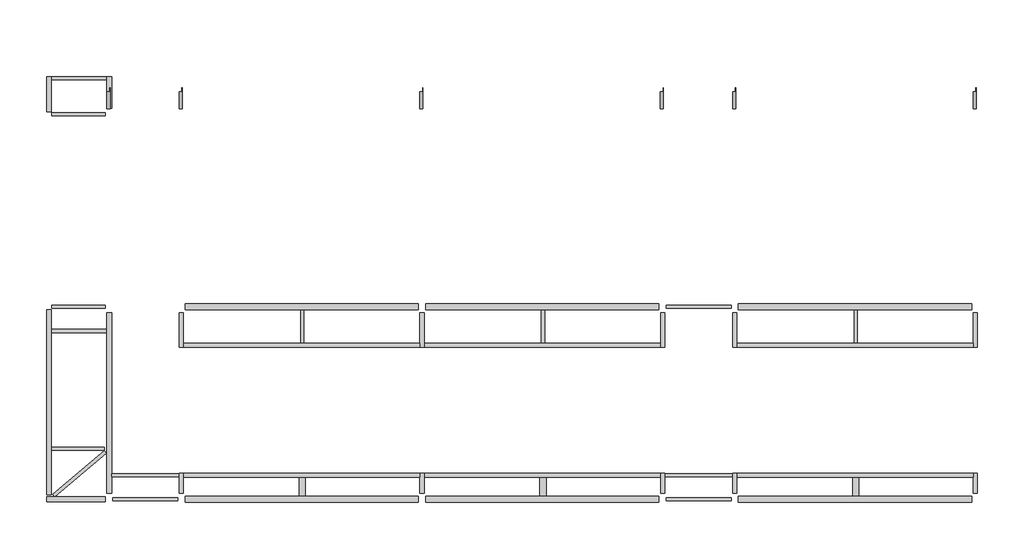
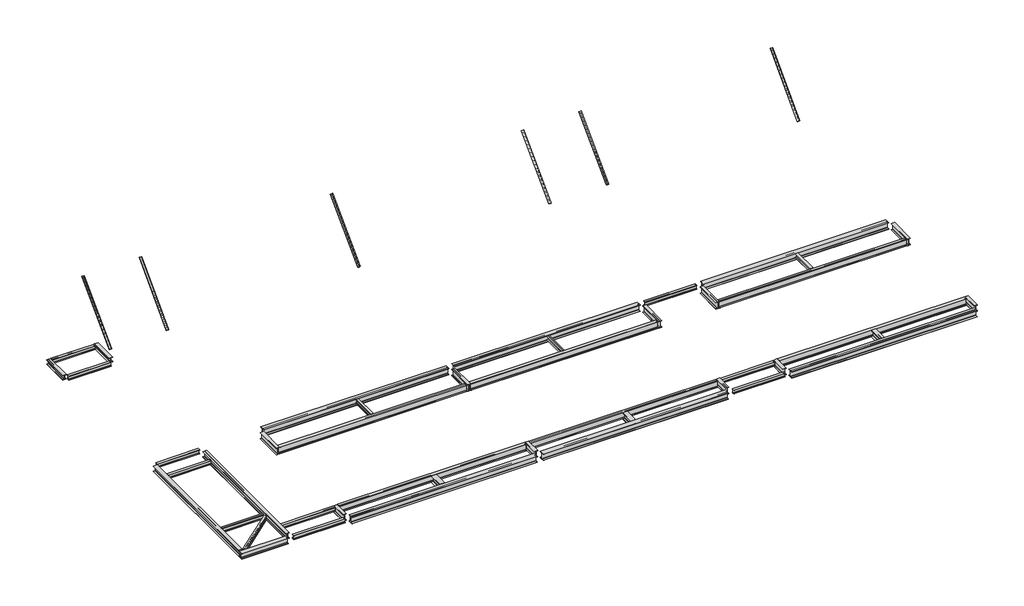
# One storey: 44 beams, 6 members.
"""IFC4 building model written with IfcOpenShell, lengths in millimetres."""

import ifcopenshell
import ifcopenshell.guid

model = None  # the IFC model being written
_history = None  # IfcOwnerHistory: only IFC2X3 demands one
_inside = {}  # id of a spatial element -> (the spatial element, [elements in it])
_under = {}  # id of a project, library or spatial element -> (it, [spatial elements below it])
_declared = {}  # id of a project -> (the project, [libraries it declares])
_typed = {}  # id of a type object -> (the type object, [elements of that type])
_made_of = {}  # id of a material, layer set ... -> (it, [elements and type objects made of it])


def new_model(schema):
    """Start an empty IFC model of exactly this schema.

    Asked for "IFC4X3", IfcOpenShell would pick the latest addendum, in which some entities
    have other attributes; the version numbers below select the first issue.
    IFC2X3 requires an IfcOwnerHistory on every rooted entity: one is made here for all.
    """
    global model, _history
    if schema == "IFC4X3":
        model = ifcopenshell.file(schema_version=(4, 3, 0, 0))
    else:
        model = ifcopenshell.file(schema=schema)
    _inside.clear()
    _under.clear()
    _declared.clear()
    _typed.clear()
    _made_of.clear()
    _history = None
    if model.schema == "IFC2X3":
        org = make("IfcOrganization", Name="unknown")
        user = make(
            "IfcPersonAndOrganization",
            ThePerson=make("IfcPerson", FamilyName="unknown"),
            TheOrganization=org,
        )
        app = make(
            "IfcApplication",
            ApplicationDeveloper=org,
            Version="unknown",
            ApplicationFullName="unknown",
            ApplicationIdentifier="unknown",
        )
        _history = make(
            "IfcOwnerHistory",
            OwningUser=user,
            OwningApplication=app,
            ChangeAction="ADDED",
            CreationDate=0,
        )
    return model


def make(cls, **values):
    """One entity of the class cls with the attributes given. An attribute that is None is left unset."""
    return model.create_entity(
        cls, **{name: value for name, value in values.items() if value is not None}
    )


def rooted(cls, **values):
    """An entity with a GlobalId (a new one), such as an element, a storey or a relation."""
    return make(cls, GlobalId=ifcopenshell.guid.new(), OwnerHistory=_history, **values)


def si_unit(unit_type, name, prefix=None):
    """IfcSIUnit, for example si_unit("LENGTHUNIT", "METRE", prefix="MILLI")."""
    return make("IfcSIUnit", UnitType=unit_type, Prefix=prefix, Name=name)


def assignment(units):
    """IfcUnitAssignment: the units of a project."""
    return None if units is None else make("IfcUnitAssignment", Units=units)


def point(xyz):
    """IfcCartesianPoint."""
    return None if xyz is None else make("IfcCartesianPoint", Coordinates=xyz)


def direction(xyz):
    """IfcDirection."""
    return None if xyz is None else make("IfcDirection", DirectionRatios=xyz)


def frame(location, z_axis=None, x_axis=None):
    """IfcAxis2Placement3D, a coordinate frame: its origin and axes. An axis left out is left unset."""
    return make(
        "IfcAxis2Placement3D",
        Location=point(location),
        Axis=direction(z_axis),
        RefDirection=direction(x_axis),
    )


def frame_2d(location, x_axis=None):
    """IfcAxis2Placement2D, a coordinate frame in the plane: its origin and x axis."""
    return make(
        "IfcAxis2Placement2D", Location=point(location), RefDirection=direction(x_axis)
    )


def origin():
    """The frame at (0, 0, 0) with its axes left unset."""
    return frame((0.0, 0.0, 0.0))


def place(relative_to, where):
    """IfcLocalPlacement: puts the frame where relative to a parent placement (None: the world)."""
    return make(
        "IfcLocalPlacement", PlacementRelTo=relative_to, RelativePlacement=where
    )


def context(
    kind, dimensions, precision=None, world=None, true_north=None, identifier=None
):
    """IfcGeometricRepresentationContext, for example the 3D "Model" context."""
    return make(
        "IfcGeometricRepresentationContext",
        ContextIdentifier=identifier,
        ContextType=kind,
        CoordinateSpaceDimension=dimensions,
        Precision=precision,
        WorldCoordinateSystem=world,
        TrueNorth=true_north,
    )


def project(units=None, contexts=None):
    """IfcProject with its units and contexts."""
    return rooted(
        "IfcProject",
        Name="project",
        RepresentationContexts=contexts,
        UnitsInContext=assignment(units),
    )


def spatial(cls, under=None, at=None, **own):
    """A site, building, storey or space (cls), placed at a placement, below another one or the project."""
    s = rooted(cls, ObjectPlacement=at, **own)
    if under is not None:
        _under.setdefault(under.id(), (under, []))[1].append(s)
    return s


def polyline(points):
    """IfcPolyline through the points."""
    return make("IfcPolyline", Points=[point(p) for p in points])


def circle_curve(where, radius):
    """IfcCircle in the frame where."""
    return make("IfcCircle", Position=where, Radius=radius)


def trimmed(basis, trim1, trim2, sense, master):
    """IfcTrimmedCurve: the piece of a basis curve between two trims."""
    return make(
        "IfcTrimmedCurve",
        BasisCurve=basis,
        Trim1=trim1,
        Trim2=trim2,
        SenseAgreement=sense,
        MasterRepresentation=master,
    )


def segment(curve, same_sense, transition):
    """IfcCompositeCurveSegment."""
    return make(
        "IfcCompositeCurveSegment",
        Transition=transition,
        SameSense=same_sense,
        ParentCurve=curve,
    )


def composite_curve(segments, self_intersect=None):
    """IfcCompositeCurve: segments joined end to end."""
    return make("IfcCompositeCurve", Segments=segments, SelfIntersect=self_intersect)


def outline(outer, holes=None, kind="AREA"):
    """IfcArbitraryClosedProfileDef: a profile drawn as a closed curve; with holes, ...WithVoids."""
    if holes is None:
        return make("IfcArbitraryClosedProfileDef", ProfileType=kind, OuterCurve=outer)
    return make(
        "IfcArbitraryProfileDefWithVoids",
        ProfileType=kind,
        OuterCurve=outer,
        InnerCurves=holes,
    )


def extrude(swept, where, along, depth):
    """IfcExtrudedAreaSolid: the profile swept, set in the frame where, extruded along a direction by depth."""
    return make(
        "IfcExtrudedAreaSolid",
        SweptArea=swept,
        Position=where,
        ExtrudedDirection=direction(along),
        Depth=depth,
    )


def shape(context_of_items, identifier, shape_type, items):
    """IfcShapeRepresentation: the items that make up one representation, for example the "Body"."""
    return make(
        "IfcShapeRepresentation",
        ContextOfItems=context_of_items,
        RepresentationIdentifier=identifier,
        RepresentationType=shape_type,
        Items=items,
    )


def source(mapping_origin, context_of_items, identifier, shape_type, items):
    """IfcRepresentationMap: a shape defined once, which mapped items show again and again."""
    return make(
        "IfcRepresentationMap",
        MappingOrigin=mapping_origin,
        MappedRepresentation=shape(context_of_items, identifier, shape_type, items),
    )


def transform(
    local_origin,
    x_axis=None,
    y_axis=None,
    z_axis=None,
    scale=None,
    scale2=None,
    scale3=None,
    uniform=True,
):
    """IfcCartesianTransformationOperator3D, or its non-uniform kind. x_axis, y_axis, z_axis: its Axis1, 2, 3."""
    if uniform:
        return make(
            "IfcCartesianTransformationOperator3D",
            Axis1=direction(x_axis),
            Axis2=direction(y_axis),
            LocalOrigin=point(local_origin),
            Scale=scale,
            Axis3=direction(z_axis),
        )
    return make(
        "IfcCartesianTransformationOperator3DnonUniform",
        Axis1=direction(x_axis),
        Axis2=direction(y_axis),
        LocalOrigin=point(local_origin),
        Scale=scale,
        Axis3=direction(z_axis),
        Scale2=scale2,
        Scale3=scale3,
    )


def mapped(mapping_source, mapping_target):
    """IfcMappedItem: shows the shape of a source again, moved by a transform."""
    return make(
        "IfcMappedItem", MappingSource=mapping_source, MappingTarget=mapping_target
    )


def made_of(thing, what):
    """Note that an element or type object is made of a material, layer set ...; save() writes the relation."""
    if what is not None:
        _made_of.setdefault(what.id(), (what, []))[1].append(thing)
    return thing


def element(
    cls,
    number,
    at=None,
    inside=None,
    cuts=None,
    type_object=None,
    material=None,
    context=None,
    identifier="Body",
    shape_type=None,
    held_by="IfcProductDefinitionShape",
    body=None,
    shapes=None,
    **own,
):
    """One element of the class cls, such as IfcWall. Its Tag is "e" and its number.

    at: its placement. inside: the storey or other place that contains it. cuts: it is an
    opening in that element (IfcRelVoidsElement). A single representation is given by context,
    identifier, shape_type and body (its items); several are given by shapes. held_by: the class
    of the entity that holds the representations. save() writes the other relations.
    """
    e = rooted(cls, Tag="e%d" % number, ObjectPlacement=at, **own)
    if body is not None:
        shapes = [shape(context, identifier, shape_type, body)]
    if shapes is not None:
        e.Representation = make(held_by, Representations=shapes)
    if inside is not None:
        _inside.setdefault(inside.id(), (inside, []))[1].append(e)
    if cuts is not None:
        rooted(
            "IfcRelVoidsElement", RelatingBuildingElement=cuts, RelatedOpeningElement=e
        )
    if type_object is not None:
        _typed.setdefault(type_object.id(), (type_object, []))[1].append(e)
    return made_of(e, material)


def aggregate(whole, parts):
    """IfcRelAggregates: a whole, such as a stair, and the parts it consists of."""
    return rooted("IfcRelAggregates", RelatingObject=whole, RelatedObjects=parts)


def save(model, path):
    """Write the relations noted so far, then the file.

    IfcRelAggregates (storeys below a building ...), IfcRelContainedInSpatialStructure (elements
    in a storey), IfcRelDefinesByType, IfcRelAssociatesMaterial and IfcRelDeclares: one each for
    every whole, place, type object, material and project.
    """
    for whole, parts in _under.values():
        aggregate(whole, parts)
    for where, things in _inside.values():
        rooted(
            "IfcRelContainedInSpatialStructure",
            RelatedElements=things,
            RelatingStructure=where,
        )
    for kind, things in _typed.values():
        rooted("IfcRelDefinesByType", RelatedObjects=things, RelatingType=kind)
    for what, things in _made_of.values():
        rooted("IfcRelAssociatesMaterial", RelatedObjects=things, RelatingMaterial=what)
    for by, libraries in _declared.values():
        rooted("IfcRelDeclares", RelatingContext=by, RelatedDefinitions=libraries)
    model.write(path)


def steel_framing_w_astm_a6m_f33feb28(model_context):
    return source(origin(), model_context, "Body", "SweptSolid", [
        extrude(outline(composite_curve([segment(polyline([(67.0, -94.8), (67.0, -105.0), (-67.0, -105.0), (-67.0, -94.8), (-10.775, -94.8)]), True, "CONTINUOUS"), segment(trimmed(circle_curve(frame_2d((-10.775, -87.2)), 7.6), [point((-10.775, -94.8))], [point((-3.175, -87.2))], True, "CARTESIAN"), True, "CONTINUOUS"), segment(polyline([(-3.175, -87.2), (-3.175, 87.2)]), True, "CONTINUOUS"), segment(trimmed(circle_curve(frame_2d((-10.775, 87.2)), 7.6), [point((-3.175, 87.2))], [point((-10.775, 94.8))], True, "CARTESIAN"), True, "CONTINUOUS"), segment(polyline([(-10.775, 94.8), (-67.0, 94.8), (-67.0, 105.0), (67.0, 105.0), (67.0, 94.8), (10.775, 94.8)]), True, "CONTINUOUS"), segment(trimmed(circle_curve(frame_2d((10.775, 87.2)), 7.6), [point((10.775, 94.8))], [point((3.175, 87.2))], True, "CARTESIAN"), True, "CONTINUOUS"), segment(polyline([(3.175, 87.2), (3.175, -87.2)]), True, "CONTINUOUS"), segment(trimmed(circle_curve(frame_2d((10.775, -87.2)), 7.6), [point((3.175, -87.2))], [point((10.775, -94.8))], True, "CARTESIAN"), True, "CONTINUOUS"), segment(polyline([(10.775, -94.8), (67.0, -94.8)]), True, "CONTINUOUS")], self_intersect=False)), frame((-1346.3, 0.0, 0.0), z_axis=(1.0, 0.0, 0.0), x_axis=(0.0, 1.0, 0.0)), (0.0, 0.0, 1.0), 2692.6),
    ])


def steel_framing_w_astm_a6m_9ad7bea0(model_context):
    return source(origin(), model_context, "Body", "SweptSolid", [
        extrude(outline(composite_curve([segment(polyline([(67.0, -94.8), (67.0, -105.0), (-67.0, -105.0), (-67.0, -94.8), (-10.775, -94.8)]), True, "CONTINUOUS"), segment(trimmed(circle_curve(frame_2d((-10.775, -87.2)), 7.6), [point((-10.775, -94.8))], [point((-3.175, -87.2))], True, "CARTESIAN"), True, "CONTINUOUS"), segment(polyline([(-3.175, -87.2), (-3.175, 87.2)]), True, "CONTINUOUS"), segment(trimmed(circle_curve(frame_2d((-10.775, 87.2)), 7.6), [point((-3.175, 87.2))], [point((-10.775, 94.8))], True, "CARTESIAN"), True, "CONTINUOUS"), segment(polyline([(-10.775, 94.8), (-67.0, 94.8), (-67.0, 105.0), (67.0, 105.0), (67.0, 94.8), (10.775, 94.8)]), True, "CONTINUOUS"), segment(trimmed(circle_curve(frame_2d((10.775, 87.2)), 7.6), [point((10.775, 94.8))], [point((3.175, 87.2))], True, "CARTESIAN"), True, "CONTINUOUS"), segment(polyline([(3.175, 87.2), (3.175, -87.2)]), True, "CONTINUOUS"), segment(trimmed(circle_curve(frame_2d((10.775, -87.2)), 7.6), [point((3.175, -87.2))], [point((10.775, -94.8))], True, "CARTESIAN"), True, "CONTINUOUS"), segment(polyline([(10.775, -94.8), (67.0, -94.8)]), True, "CONTINUOUS")], self_intersect=False)), frame((-1135.3, 0.0, 0.0), z_axis=(1.0, 0.0, 0.0), x_axis=(0.0, 1.0, 0.0)), (0.0, 0.0, 1.0), 2231.6),
    ])


def steel_framing_w_astm_a6m_5f95f2a9(model_context):
    return source(origin(), model_context, "Body", "SweptSolid", [
        extrude(outline(composite_curve([segment(polyline([(67.0, -94.8), (67.0, -105.0), (-67.0, -105.0), (-67.0, -94.8), (-10.775, -94.8)]), True, "CONTINUOUS"), segment(trimmed(circle_curve(frame_2d((-10.775, -87.2)), 7.6), [point((-10.775, -94.8))], [point((-3.175, -87.2))], True, "CARTESIAN"), True, "CONTINUOUS"), segment(polyline([(-3.175, -87.2), (-3.175, 87.2)]), True, "CONTINUOUS"), segment(trimmed(circle_curve(frame_2d((-10.775, 87.2)), 7.6), [point((-3.175, 87.2))], [point((-10.775, 94.8))], True, "CARTESIAN"), True, "CONTINUOUS"), segment(polyline([(-10.775, 94.8), (-67.0, 94.8), (-67.0, 105.0), (67.0, 105.0), (67.0, 94.8), (10.775, 94.8)]), True, "CONTINUOUS"), segment(trimmed(circle_curve(frame_2d((10.775, 87.2)), 7.6), [point((10.775, 94.8))], [point((3.175, 87.2))], True, "CARTESIAN"), True, "CONTINUOUS"), segment(polyline([(3.175, 87.2), (3.175, -87.2)]), True, "CONTINUOUS"), segment(trimmed(circle_curve(frame_2d((10.775, -87.2)), 7.6), [point((3.175, -87.2))], [point((10.775, -94.8))], True, "CARTESIAN"), True, "CONTINUOUS"), segment(polyline([(10.775, -94.8), (67.0, -94.8)]), True, "CONTINUOUS")], self_intersect=False)), frame((-1401.8, 0.0, 0.0), z_axis=(1.0, 0.0, 0.0), x_axis=(0.0, 1.0, 0.0)), (0.0, 0.0, 1.0), 2803.6),
    ])


def steel_framing_w_astm_a6m_17837fc5(model_context):
    return source(origin(), model_context, "Body", "SweptSolid", [
        extrude(outline(composite_curve([segment(polyline([(127.0, -160.1), (127.0, -176.5), (-127.0, -176.5), (-127.0, -160.1), (-19.865, -160.1)]), True, "CONTINUOUS"), segment(trimmed(circle_curve(frame_2d((-19.865, -145.0)), 15.1), [point((-19.865, -160.1))], [point((-4.765, -145.0))], True, "CARTESIAN"), True, "CONTINUOUS"), segment(polyline([(-4.765, -145.0), (-4.765, 145.0)]), True, "CONTINUOUS"), segment(trimmed(circle_curve(frame_2d((-19.865, 145.0)), 15.1), [point((-4.765, 145.0))], [point((-19.865, 160.1))], True, "CARTESIAN"), True, "CONTINUOUS"), segment(polyline([(-19.865, 160.1), (-127.0, 160.1), (-127.0, 176.5), (127.0, 176.5), (127.0, 160.1), (19.865, 160.1)]), True, "CONTINUOUS"), segment(trimmed(circle_curve(frame_2d((19.865, 145.0)), 15.1), [point((19.865, 160.1))], [point((4.765, 145.0))], True, "CARTESIAN"), True, "CONTINUOUS"), segment(polyline([(4.765, 145.0), (4.765, -145.0)]), True, "CONTINUOUS"), segment(trimmed(circle_curve(frame_2d((19.865, -145.0)), 15.1), [point((4.765, -145.0))], [point((19.865, -160.1))], True, "CARTESIAN"), True, "CONTINUOUS"), segment(polyline([(19.865, -160.1), (127.0, -160.1)]), True, "CONTINUOUS")], self_intersect=False)), frame((-4846.3, 0.0, 0.0), z_axis=(1.0, 0.0, 0.0), x_axis=(0.0, 1.0, 0.0)), (0.0, 0.0, 1.0), 9692.6),
    ])


def steel_framing_w_astm_a6m_8cea9429(model_context):
    return source(origin(), model_context, "Body", "SweptSolid", [
        extrude(outline(composite_curve([segment(polyline([(101.5, -137.9), (101.5, -151.0), (-101.5, -151.0), (-101.5, -137.9), (-16.545, -137.9)]), True, "CONTINUOUS"), segment(trimmed(circle_curve(frame_2d((-16.545, -125.1)), 12.8), [point((-16.545, -137.9))], [point((-3.745, -125.1))], True, "CARTESIAN"), True, "CONTINUOUS"), segment(polyline([(-3.745, -125.1), (-3.745, 125.1)]), True, "CONTINUOUS"), segment(trimmed(circle_curve(frame_2d((-16.545, 125.1)), 12.8), [point((-3.745, 125.1))], [point((-16.545, 137.9))], True, "CARTESIAN"), True, "CONTINUOUS"), segment(polyline([(-16.545, 137.9), (-101.5, 137.9), (-101.5, 151.0), (101.5, 151.0), (101.5, 137.9), (16.545, 137.9)]), True, "CONTINUOUS"), segment(trimmed(circle_curve(frame_2d((16.545, 125.1)), 12.8), [point((16.545, 137.9))], [point((3.745, 125.1))], True, "CARTESIAN"), True, "CONTINUOUS"), segment(polyline([(3.745, 125.1), (3.745, -125.1)]), True, "CONTINUOUS"), segment(trimmed(circle_curve(frame_2d((16.545, -125.1)), 12.8), [point((3.745, -125.1))], [point((16.545, -137.9))], True, "CARTESIAN"), True, "CONTINUOUS"), segment(polyline([(16.545, -137.9), (101.5, -137.9)]), True, "CONTINUOUS")], self_intersect=False)), frame((-3753.8, 0.0, 0.0), z_axis=(1.0, 0.0, 0.0), x_axis=(0.0, 1.0, 0.0)), (0.0, 0.0, 1.0), 7507.6),
    ])


def steel_framing_w_astm_a6m_ee6b765e(model_context):
    return source(origin(), model_context, "Body", "SweptSolid", [
        extrude(outline(composite_curve([segment(polyline([(101.0, -112.5), (101.0, -123.5), (-101.0, -123.5), (-101.0, -112.5), (-16.385, -112.5)]), True, "CONTINUOUS"), segment(trimmed(circle_curve(frame_2d((-16.385, -99.8)), 12.7), [point((-16.385, -112.5))], [point((-3.685, -99.8))], True, "CARTESIAN"), True, "CONTINUOUS"), segment(polyline([(-3.685, -99.8), (-3.685, 99.8)]), True, "CONTINUOUS"), segment(trimmed(circle_curve(frame_2d((-16.385, 99.8)), 12.7), [point((-3.685, 99.8))], [point((-16.385, 112.5))], True, "CARTESIAN"), True, "CONTINUOUS"), segment(polyline([(-16.385, 112.5), (-101.0, 112.5), (-101.0, 123.5), (101.0, 123.5), (101.0, 112.5), (16.385, 112.5)]), True, "CONTINUOUS"), segment(trimmed(circle_curve(frame_2d((16.385, 99.8)), 12.7), [point((16.385, 112.5))], [point((3.685, 99.8))], True, "CARTESIAN"), True, "CONTINUOUS"), segment(polyline([(3.685, 99.8), (3.685, -99.8)]), True, "CONTINUOUS"), segment(trimmed(circle_curve(frame_2d((16.385, -99.8)), 12.7), [point((3.685, -99.8))], [point((16.385, -112.5))], True, "CARTESIAN"), True, "CONTINUOUS"), segment(polyline([(16.385, -112.5), (101.0, -112.5)]), True, "CONTINUOUS")], self_intersect=False)), frame((-634.3, 0.0, 0.0), z_axis=(1.0, 0.0, 0.0), x_axis=(0.0, 1.0, 0.0)), (0.0, 0.0, 1.0), 1451.3),
    ])


def steel_framing_w_astm_a6m_8355ed91(model_context):
    return source(origin(), model_context, "Body", "SweptSolid", [
        extrude(outline(composite_curve([segment(polyline([(67.0, -94.8), (67.0, -105.0), (-67.0, -105.0), (-67.0, -94.8), (-10.775, -94.8)]), True, "CONTINUOUS"), segment(trimmed(circle_curve(frame_2d((-10.775, -87.2)), 7.6), [point((-10.775, -94.8))], [point((-3.175, -87.2))], True, "CARTESIAN"), True, "CONTINUOUS"), segment(polyline([(-3.175, -87.2), (-3.175, 87.2)]), True, "CONTINUOUS"), segment(trimmed(circle_curve(frame_2d((-10.775, 87.2)), 7.6), [point((-3.175, 87.2))], [point((-10.775, 94.8))], True, "CARTESIAN"), True, "CONTINUOUS"), segment(polyline([(-10.775, 94.8), (-67.0, 94.8), (-67.0, 105.0), (67.0, 105.0), (67.0, 94.8), (10.775, 94.8)]), True, "CONTINUOUS"), segment(trimmed(circle_curve(frame_2d((10.775, 87.2)), 7.6), [point((10.775, 94.8))], [point((3.175, 87.2))], True, "CARTESIAN"), True, "CONTINUOUS"), segment(polyline([(3.175, 87.2), (3.175, -87.2)]), True, "CONTINUOUS"), segment(trimmed(circle_curve(frame_2d((10.775, -87.2)), 7.6), [point((3.175, -87.2))], [point((10.775, -94.8))], True, "CARTESIAN"), True, "CONTINUOUS"), segment(polyline([(10.775, -94.8), (67.0, -94.8)]), True, "CONTINUOUS")], self_intersect=False)), frame((-1136.3, 0.0, 0.0), z_axis=(1.0, 0.0, 0.0), x_axis=(0.0, 1.0, 0.0)), (0.0, 0.0, 1.0), 2272.6),
    ])


def steel_framing_w_astm_a6m_7f0d9279(model_context):
    return source(origin(), model_context, "Body", "SweptSolid", [
        extrude(outline(composite_curve([segment(polyline([(101.0, -112.5), (101.0, -123.5), (-101.0, -123.5), (-101.0, -112.5), (-16.385, -112.5)]), True, "CONTINUOUS"), segment(trimmed(circle_curve(frame_2d((-16.385, -99.8)), 12.7), [point((-16.385, -112.5))], [point((-3.685, -99.8))], True, "CARTESIAN"), True, "CONTINUOUS"), segment(polyline([(-3.685, -99.8), (-3.685, 99.8)]), True, "CONTINUOUS"), segment(trimmed(circle_curve(frame_2d((-16.385, 99.8)), 12.7), [point((-3.685, 99.8))], [point((-16.385, 112.5))], True, "CARTESIAN"), True, "CONTINUOUS"), segment(polyline([(-16.385, 112.5), (-101.0, 112.5), (-101.0, 123.5), (101.0, 123.5), (101.0, 112.5), (16.385, 112.5)]), True, "CONTINUOUS"), segment(trimmed(circle_curve(frame_2d((16.385, 99.8)), 12.7), [point((16.385, 112.5))], [point((3.685, 99.8))], True, "CARTESIAN"), True, "CONTINUOUS"), segment(polyline([(3.685, 99.8), (3.685, -99.8)]), True, "CONTINUOUS"), segment(trimmed(circle_curve(frame_2d((16.385, -99.8)), 12.7), [point((3.685, -99.8))], [point((16.385, -112.5))], True, "CARTESIAN"), True, "CONTINUOUS"), segment(polyline([(16.385, -112.5), (101.0, -112.5)]), True, "CONTINUOUS")], self_intersect=False)), frame((-503.8, 0.0, 0.0), z_axis=(1.0, 0.0, 0.0), x_axis=(0.0, 1.0, 0.0)), (0.0, 0.0, 1.0), 1320.8),
    ])


def steel_framing_w_astm_a6m_9f313648(model_context):
    return source(origin(), model_context, "Body", "SweptSolid", [
        extrude(outline(composite_curve([segment(polyline([(67.0, -94.8), (67.0, -105.0), (-67.0, -105.0), (-67.0, -94.8), (-10.775, -94.8)]), True, "CONTINUOUS"), segment(trimmed(circle_curve(frame_2d((-10.775, -87.2)), 7.6), [point((-10.775, -94.8))], [point((-3.175, -87.2))], True, "CARTESIAN"), True, "CONTINUOUS"), segment(polyline([(-3.175, -87.2), (-3.175, 87.2)]), True, "CONTINUOUS"), segment(trimmed(circle_curve(frame_2d((-10.775, 87.2)), 7.6), [point((-3.175, 87.2))], [point((-10.775, 94.8))], True, "CARTESIAN"), True, "CONTINUOUS"), segment(polyline([(-10.775, 94.8), (-67.0, 94.8), (-67.0, 105.0), (67.0, 105.0), (67.0, 94.8), (10.775, 94.8)]), True, "CONTINUOUS"), segment(trimmed(circle_curve(frame_2d((10.775, 87.2)), 7.6), [point((10.775, 94.8))], [point((3.175, 87.2))], True, "CARTESIAN"), True, "CONTINUOUS"), segment(polyline([(3.175, 87.2), (3.175, -87.2)]), True, "CONTINUOUS"), segment(trimmed(circle_curve(frame_2d((10.775, -87.2)), 7.6), [point((3.175, -87.2))], [point((10.775, -94.8))], True, "CARTESIAN"), True, "CONTINUOUS"), segment(polyline([(10.775, -94.8), (67.0, -94.8)]), True, "CONTINUOUS")], self_intersect=False)), frame((-1135.8, 0.0, 0.0), z_axis=(1.0, 0.0, 0.0), x_axis=(0.0, 1.0, 0.0)), (0.0, 0.0, 1.0), 2271.6),
    ])


def steel_framing_w_astm_a6m_8815720a(model_context):
    return source(origin(), model_context, "Body", "SweptSolid", [
        extrude(outline(composite_curve([segment(polyline([(101.5, -137.9), (101.5, -151.0), (-101.5, -151.0), (-101.5, -137.9), (-16.545, -137.9)]), True, "CONTINUOUS"), segment(trimmed(circle_curve(frame_2d((-16.545, -125.1)), 12.8), [point((-16.545, -137.9))], [point((-3.745, -125.1))], True, "CARTESIAN"), True, "CONTINUOUS"), segment(polyline([(-3.745, -125.1), (-3.745, 125.1)]), True, "CONTINUOUS"), segment(trimmed(circle_curve(frame_2d((-16.545, 125.1)), 12.8), [point((-3.745, 125.1))], [point((-16.545, 137.9))], True, "CARTESIAN"), True, "CONTINUOUS"), segment(polyline([(-16.545, 137.9), (-101.5, 137.9), (-101.5, 151.0), (101.5, 151.0), (101.5, 137.9), (16.545, 137.9)]), True, "CONTINUOUS"), segment(trimmed(circle_curve(frame_2d((16.545, 125.1)), 12.8), [point((16.545, 137.9))], [point((3.745, 125.1))], True, "CARTESIAN"), True, "CONTINUOUS"), segment(polyline([(3.745, 125.1), (3.745, -125.1)]), True, "CONTINUOUS"), segment(trimmed(circle_curve(frame_2d((16.545, -125.1)), 12.8), [point((3.745, -125.1))], [point((16.545, -137.9))], True, "CARTESIAN"), True, "CONTINUOUS"), segment(polyline([(16.545, -137.9), (101.5, -137.9)]), True, "CONTINUOUS")], self_intersect=False)), frame((-1096.3, 0.0, 0.0), z_axis=(1.0, 0.0, 0.0), x_axis=(0.0, 1.0, 0.0)), (0.0, 0.0, 1.0), 2447.8),
    ])


def steel_framing_w_astm_a6m_1b426b15(model_context):
    return source(origin(), model_context, "Body", "SweptSolid", [
        extrude(outline(composite_curve([segment(polyline([(67.0, -94.8), (67.0, -105.0), (-67.0, -105.0), (-67.0, -94.8), (-10.775, -94.8)]), True, "CONTINUOUS"), segment(trimmed(circle_curve(frame_2d((-10.775, -87.2)), 7.6), [point((-10.775, -94.8))], [point((-3.175, -87.2))], True, "CARTESIAN"), True, "CONTINUOUS"), segment(polyline([(-3.175, -87.2), (-3.175, 87.2)]), True, "CONTINUOUS"), segment(trimmed(circle_curve(frame_2d((-10.775, 87.2)), 7.6), [point((-3.175, 87.2))], [point((-10.775, 94.8))], True, "CARTESIAN"), True, "CONTINUOUS"), segment(polyline([(-10.775, 94.8), (-67.0, 94.8), (-67.0, 105.0), (67.0, 105.0), (67.0, 94.8), (10.775, 94.8)]), True, "CONTINUOUS"), segment(trimmed(circle_curve(frame_2d((10.775, 87.2)), 7.6), [point((10.775, 94.8))], [point((3.175, 87.2))], True, "CARTESIAN"), True, "CONTINUOUS"), segment(polyline([(3.175, 87.2), (3.175, -87.2)]), True, "CONTINUOUS"), segment(trimmed(circle_curve(frame_2d((10.775, -87.2)), 7.6), [point((3.175, -87.2))], [point((10.775, -94.8))], True, "CARTESIAN"), True, "CONTINUOUS"), segment(polyline([(10.775, -94.8), (67.0, -94.8)]), True, "CONTINUOUS")], self_intersect=False)), frame((-1135.8, 0.0, 0.0), z_axis=(1.0, 0.0, 0.0), x_axis=(0.0, 1.0, 0.0)), (0.0, 0.0, 1.0), 2189.1),
    ])


def steel_framing_w_astm_a6m_97b597d5(model_context):
    return source(origin(), model_context, "Body", "SweptSolid", [
        extrude(outline(composite_curve([segment(polyline([(101.5, -137.9), (101.5, -151.0), (-101.5, -151.0), (-101.5, -137.9), (-16.545, -137.9)]), True, "CONTINUOUS"), segment(trimmed(circle_curve(frame_2d((-16.545, -125.1)), 12.8), [point((-16.545, -137.9))], [point((-3.745, -125.1))], True, "CARTESIAN"), True, "CONTINUOUS"), segment(polyline([(-3.745, -125.1), (-3.745, 125.1)]), True, "CONTINUOUS"), segment(trimmed(circle_curve(frame_2d((-16.545, 125.1)), 12.8), [point((-3.745, 125.1))], [point((-16.545, 137.9))], True, "CARTESIAN"), True, "CONTINUOUS"), segment(polyline([(-16.545, 137.9), (-101.5, 137.9), (-101.5, 151.0), (101.5, 151.0), (101.5, 137.9), (16.545, 137.9)]), True, "CONTINUOUS"), segment(trimmed(circle_curve(frame_2d((16.545, 125.1)), 12.8), [point((16.545, 137.9))], [point((3.745, 125.1))], True, "CARTESIAN"), True, "CONTINUOUS"), segment(polyline([(3.745, 125.1), (3.745, -125.1)]), True, "CONTINUOUS"), segment(trimmed(circle_curve(frame_2d((16.545, -125.1)), 12.8), [point((3.745, -125.1))], [point((16.545, -137.9))], True, "CARTESIAN"), True, "CONTINUOUS"), segment(polyline([(16.545, -137.9), (101.5, -137.9)]), True, "CONTINUOUS")], self_intersect=False)), frame((-3884.3, 0.0, 0.0), z_axis=(1.0, 0.0, 0.0), x_axis=(0.0, 1.0, 0.0)), (0.0, 0.0, 1.0), 7698.8),
    ])


def steel_framing_w_astm_a6m_8d3d16c6(model_context):
    return source(origin(), model_context, "Body", "SweptSolid", [
        extrude(outline(composite_curve([segment(polyline([(67.0, -94.8), (67.0, -105.0), (-67.0, -105.0), (-67.0, -94.8), (-10.775, -94.8)]), True, "CONTINUOUS"), segment(trimmed(circle_curve(frame_2d((-10.775, -87.2)), 7.6), [point((-10.775, -94.8))], [point((-3.175, -87.2))], True, "CARTESIAN"), True, "CONTINUOUS"), segment(polyline([(-3.175, -87.2), (-3.175, 87.2)]), True, "CONTINUOUS"), segment(trimmed(circle_curve(frame_2d((-10.775, 87.2)), 7.6), [point((-3.175, 87.2))], [point((-10.775, 94.8))], True, "CARTESIAN"), True, "CONTINUOUS"), segment(polyline([(-10.775, 94.8), (-67.0, 94.8), (-67.0, 105.0), (67.0, 105.0), (67.0, 94.8), (10.775, 94.8)]), True, "CONTINUOUS"), segment(trimmed(circle_curve(frame_2d((10.775, 87.2)), 7.6), [point((10.775, 94.8))], [point((3.175, 87.2))], True, "CARTESIAN"), True, "CONTINUOUS"), segment(polyline([(3.175, 87.2), (3.175, -87.2)]), True, "CONTINUOUS"), segment(trimmed(circle_curve(frame_2d((10.775, -87.2)), 7.6), [point((3.175, -87.2))], [point((10.775, -94.8))], True, "CARTESIAN"), True, "CONTINUOUS"), segment(polyline([(10.775, -94.8), (67.0, -94.8)]), True, "CONTINUOUS")], self_intersect=False)), frame((-1382.2, 0.0, 0.0), z_axis=(1.0, 0.0, 0.0), x_axis=(0.0, 1.0, 0.0)), (0.0, 0.0, 1.0), 2813.1),
    ])


def steel_framing_w_astm_a6m_0a69f8b6(model_context):
    return source(origin(), model_context, "Body", "SweptSolid", [
        extrude(outline(composite_curve([segment(polyline([(67.0, -94.8), (67.0, -105.0), (-67.0, -105.0), (-67.0, -94.8), (-10.775, -94.8)]), True, "CONTINUOUS"), segment(trimmed(circle_curve(frame_2d((-10.775, -87.2)), 7.6), [point((-10.775, -94.8))], [point((-3.175, -87.2))], True, "CARTESIAN"), True, "CONTINUOUS"), segment(polyline([(-3.175, -87.2), (-3.175, 87.2)]), True, "CONTINUOUS"), segment(trimmed(circle_curve(frame_2d((-10.775, 87.2)), 7.6), [point((-3.175, 87.2))], [point((-10.775, 94.8))], True, "CARTESIAN"), True, "CONTINUOUS"), segment(polyline([(-10.775, 94.8), (-67.0, 94.8), (-67.0, 105.0), (67.0, 105.0), (67.0, 94.8), (10.775, 94.8)]), True, "CONTINUOUS"), segment(trimmed(circle_curve(frame_2d((10.775, 87.2)), 7.6), [point((10.775, 94.8))], [point((3.175, 87.2))], True, "CARTESIAN"), True, "CONTINUOUS"), segment(polyline([(3.175, 87.2), (3.175, -87.2)]), True, "CONTINUOUS"), segment(trimmed(circle_curve(frame_2d((10.775, -87.2)), 7.6), [point((3.175, -87.2))], [point((10.775, -94.8))], True, "CARTESIAN"), True, "CONTINUOUS"), segment(polyline([(10.775, -94.8), (67.0, -94.8)]), True, "CONTINUOUS")], self_intersect=False)), frame((-1385.8, 0.0, 0.0), z_axis=(1.0, 0.0, 0.0), x_axis=(0.0, 1.0, 0.0)), (0.0, 0.0, 1.0), 2787.6),
    ])


def steel_framing_w_astm_a6m_0f62209b(model_context):
    return source(origin(), model_context, "Body", "SweptSolid", [
        extrude(outline(composite_curve([segment(polyline([(85.5, -166.4), (85.5, -178.0), (-85.5, -178.0), (-85.5, -166.4), (-13.72, -166.4)]), True, "CONTINUOUS"), segment(trimmed(circle_curve(frame_2d((-13.72, -156.3)), 10.1), [point((-13.72, -166.4))], [point((-3.62, -156.3))], True, "CARTESIAN"), True, "CONTINUOUS"), segment(polyline([(-3.62, -156.3), (-3.62, 156.3)]), True, "CONTINUOUS"), segment(trimmed(circle_curve(frame_2d((-13.72, 156.3)), 10.1), [point((-3.62, 156.3))], [point((-13.72, 166.4))], True, "CARTESIAN"), True, "CONTINUOUS"), segment(polyline([(-13.72, 166.4), (-85.5, 166.4), (-85.5, 178.0), (85.5, 178.0), (85.5, 166.4), (13.72, 166.4)]), True, "CONTINUOUS"), segment(trimmed(circle_curve(frame_2d((13.72, 156.3)), 10.1), [point((13.72, 166.4))], [point((3.62, 156.3))], True, "CARTESIAN"), True, "CONTINUOUS"), segment(polyline([(3.62, 156.3), (3.62, -156.3)]), True, "CONTINUOUS"), segment(trimmed(circle_curve(frame_2d((13.72, -156.3)), 10.1), [point((3.62, -156.3))], [point((13.72, -166.4))], True, "CARTESIAN"), True, "CONTINUOUS"), segment(polyline([(13.72, -166.4), (85.5, -166.4)]), True, "CONTINUOUS")], self_intersect=False)), frame((-253.8, 0.0, 0.0), z_axis=(1.0, 0.0, 0.0), x_axis=(0.0, 1.0, 0.0)), (0.0, 0.0, 1.0), 839.3),
    ])


def steel_framing_w_astm_a6m_8e55c2dc(model_context):
    return source(origin(), model_context, "Body", "SweptSolid", [
        extrude(outline(composite_curve([segment(polyline([(85.5, -166.4), (85.5, -178.0), (-85.5, -178.0), (-85.5, -166.4), (-13.72, -166.4)]), True, "CONTINUOUS"), segment(trimmed(circle_curve(frame_2d((-13.72, -156.3)), 10.1), [point((-13.72, -166.4))], [point((-3.62, -156.3))], True, "CARTESIAN"), True, "CONTINUOUS"), segment(polyline([(-3.62, -156.3), (-3.62, 156.3)]), True, "CONTINUOUS"), segment(trimmed(circle_curve(frame_2d((-13.72, 156.3)), 10.1), [point((-3.62, 156.3))], [point((-13.72, 166.4))], True, "CARTESIAN"), True, "CONTINUOUS"), segment(polyline([(-13.72, 166.4), (-85.5, 166.4), (-85.5, 178.0), (85.5, 178.0), (85.5, 166.4), (13.72, 166.4)]), True, "CONTINUOUS"), segment(trimmed(circle_curve(frame_2d((13.72, 156.3)), 10.1), [point((13.72, 166.4))], [point((3.62, 156.3))], True, "CARTESIAN"), True, "CONTINUOUS"), segment(polyline([(3.62, 156.3), (3.62, -156.3)]), True, "CONTINUOUS"), segment(trimmed(circle_curve(frame_2d((13.72, -156.3)), 10.1), [point((3.62, -156.3))], [point((13.72, -166.4))], True, "CARTESIAN"), True, "CONTINUOUS"), segment(polyline([(13.72, -166.4), (85.5, -166.4)]), True, "CONTINUOUS")], self_intersect=False)), frame((-4901.8, 0.0, 0.0), z_axis=(1.0, 0.0, 0.0), x_axis=(0.0, 1.0, 0.0)), (0.0, 0.0, 1.0), 9803.6),
    ])


def steel_framing_w_astm_a6m_0ec37d14(model_context):
    return source(origin(), model_context, "Body", "SweptSolid", [
        extrude(outline(composite_curve([segment(polyline([(85.5, -166.4), (85.5, -178.0), (-85.5, -178.0), (-85.5, -166.4), (-13.72, -166.4)]), True, "CONTINUOUS"), segment(trimmed(circle_curve(frame_2d((-13.72, -156.3)), 10.1), [point((-13.72, -166.4))], [point((-3.62, -156.3))], True, "CARTESIAN"), True, "CONTINUOUS"), segment(polyline([(-3.62, -156.3), (-3.62, 156.3)]), True, "CONTINUOUS"), segment(trimmed(circle_curve(frame_2d((-13.72, 156.3)), 10.1), [point((-3.62, 156.3))], [point((-13.72, 166.4))], True, "CARTESIAN"), True, "CONTINUOUS"), segment(polyline([(-13.72, 166.4), (-85.5, 166.4), (-85.5, 178.0), (85.5, 178.0), (85.5, 166.4), (13.72, 166.4)]), True, "CONTINUOUS"), segment(trimmed(circle_curve(frame_2d((13.72, 156.3)), 10.1), [point((13.72, 166.4))], [point((3.62, 156.3))], True, "CARTESIAN"), True, "CONTINUOUS"), segment(polyline([(3.62, 156.3), (3.62, -156.3)]), True, "CONTINUOUS"), segment(trimmed(circle_curve(frame_2d((13.72, -156.3)), 10.1), [point((3.62, -156.3))], [point((13.72, -166.4))], True, "CARTESIAN"), True, "CONTINUOUS"), segment(polyline([(13.72, -166.4), (85.5, -166.4)]), True, "CONTINUOUS")], self_intersect=False)), frame((-553.8, 0.0, 0.0), z_axis=(1.0, 0.0, 0.0), x_axis=(0.0, 1.0, 0.0)), (0.0, 0.0, 1.0), 1439.3),
    ])


def steel_framing_w_astm_a6m_e50dfa28(model_context):
    return source(origin(), model_context, "Body", "SweptSolid", [
        extrude(outline(composite_curve([segment(polyline([(67.0, -94.8), (67.0, -105.0), (-67.0, -105.0), (-67.0, -94.8), (-10.775, -94.8)]), True, "CONTINUOUS"), segment(trimmed(circle_curve(frame_2d((-10.775, -87.2)), 7.6), [point((-10.775, -94.8))], [point((-3.175, -87.2))], True, "CARTESIAN"), True, "CONTINUOUS"), segment(polyline([(-3.175, -87.2), (-3.175, 87.2)]), True, "CONTINUOUS"), segment(trimmed(circle_curve(frame_2d((-10.775, 87.2)), 7.6), [point((-3.175, 87.2))], [point((-10.775, 94.8))], True, "CARTESIAN"), True, "CONTINUOUS"), segment(polyline([(-10.775, 94.8), (-67.0, 94.8), (-67.0, 105.0), (67.0, 105.0), (67.0, 94.8), (10.775, 94.8)]), True, "CONTINUOUS"), segment(trimmed(circle_curve(frame_2d((10.775, 87.2)), 7.6), [point((10.775, 94.8))], [point((3.175, 87.2))], True, "CARTESIAN"), True, "CONTINUOUS"), segment(polyline([(3.175, 87.2), (3.175, -87.2)]), True, "CONTINUOUS"), segment(trimmed(circle_curve(frame_2d((10.775, -87.2)), 7.6), [point((3.175, -87.2))], [point((10.775, -94.8))], True, "CARTESIAN"), True, "CONTINUOUS"), segment(polyline([(10.775, -94.8), (67.0, -94.8)]), True, "CONTINUOUS")], self_intersect=False)), frame((-660.3, 0.0, 0.0), z_axis=(1.0, 0.0, 0.0), x_axis=(0.0, 1.0, 0.0)), (0.0, 0.0, 1.0), 1362.1),
    ])


def steel_framing_w_astm_a6m_e4d07942(model_context):
    return source(origin(), model_context, "Body", "SweptSolid", [
        extrude(outline(composite_curve([segment(polyline([(127.0, -160.1), (127.0, -176.5), (-127.0, -176.5), (-127.0, -160.1), (-19.865, -160.1)]), True, "CONTINUOUS"), segment(trimmed(circle_curve(frame_2d((-19.865, -145.0)), 15.1), [point((-19.865, -160.1))], [point((-4.765, -145.0))], True, "CARTESIAN"), True, "CONTINUOUS"), segment(polyline([(-4.765, -145.0), (-4.765, 145.0)]), True, "CONTINUOUS"), segment(trimmed(circle_curve(frame_2d((-19.865, 145.0)), 15.1), [point((-4.765, 145.0))], [point((-19.865, 160.1))], True, "CARTESIAN"), True, "CONTINUOUS"), segment(polyline([(-19.865, 160.1), (-127.0, 160.1), (-127.0, 176.5), (127.0, 176.5), (127.0, 160.1), (19.865, 160.1)]), True, "CONTINUOUS"), segment(trimmed(circle_curve(frame_2d((19.865, 145.0)), 15.1), [point((19.865, 160.1))], [point((4.765, 145.0))], True, "CARTESIAN"), True, "CONTINUOUS"), segment(polyline([(4.765, 145.0), (4.765, -145.0)]), True, "CONTINUOUS"), segment(trimmed(circle_curve(frame_2d((19.865, -145.0)), 15.1), [point((4.765, -145.0))], [point((19.865, -160.1))], True, "CARTESIAN"), True, "CONTINUOUS"), segment(polyline([(19.865, -160.1), (127.0, -160.1)]), True, "CONTINUOUS")], self_intersect=False)), frame((-360.3, 0.0, 0.0), z_axis=(1.0, 0.0, 0.0), x_axis=(0.0, 1.0, 0.0)), (0.0, 0.0, 1.0), 762.1),
    ])


def member_14297e1c(model_context):
    return source(origin(), model_context, "Body", "SweptSolid", [
        extrude(outline(composite_curve([segment(polyline([(36.4, 36.4), (36.4, -93.6)]), True, "CONTINUOUS"), segment(trimmed(circle_curve(frame_2d((36.4, -81.6)), 12.0), [point((36.4, -93.6))], [point((24.4, -81.6))], False, "CARTESIAN"), True, "CONTINUOUS"), segment(polyline([(24.4, -81.6), (24.4, 12.4)]), True, "CONTINUOUS"), segment(trimmed(circle_curve(frame_2d((12.4, 12.4)), 12.0), [point((24.4, 12.4))], [point((12.4, 24.4))], True, "CARTESIAN"), True, "CONTINUOUS"), segment(polyline([(12.4, 24.4), (-81.6, 24.4)]), True, "CONTINUOUS"), segment(trimmed(circle_curve(frame_2d((-81.6, 36.4)), 12.0), [point((-81.6, 24.4))], [point((-93.6, 36.4))], False, "CARTESIAN"), True, "CONTINUOUS"), segment(polyline([(-93.6, 36.4), (36.4, 36.4)]), True, "CONTINUOUS")], self_intersect=False)), frame((-1819.863551, 0.0, 0.0), z_axis=(1.0, 0.0, 0.0), x_axis=(0.0, 1.0, 0.0)), (0.0, 0.0, 1.0), 3551.9244278),
    ])


model = new_model("IFC4")

# Units and contexts
model_context = context("Model", 3, world=origin())
ifc_project = project(units=[si_unit("LENGTHUNIT", "METRE", prefix="MILLI")], contexts=[model_context])

# Site, building, storey
site = spatial("IfcSite", under=ifc_project)
building = spatial("IfcBuilding", under=site)
storey = spatial("IfcBuildingStorey", under=building, Name="T.O.S(2-1)", Elevation=519.8243501)

# Beams
placement = place(None, origin())
steel_framing_w_astm_a6m_shape = steel_framing_w_astm_a6m_f33feb28(model_context)
element("IfcBeam", 1, ObjectType="Steel Framing_W_ASTM A6M", at=placement, inside=storey, context=model_context, shape_type="MappedRepresentation", body=[
    mapped(steel_framing_w_astm_a6m_shape, transform((1500.0, 6499.5208589, 414.8243501), x_axis=(1.0, 0.0, 0.0), y_axis=(0.0, 1.0, 0.0), z_axis=(0.0, 0.0, 1.0))),
])
element("IfcBeam", 2, ObjectType="Steel Framing_W_ASTM A6M", at=placement, inside=storey, context=model_context, shape_type="MappedRepresentation", body=[
    mapped(steel_framing_w_astm_a6m_shape, transform((24500.0, 6499.5208589, 414.8243501), x_axis=(1.0, 0.0, 0.0), y_axis=(0.0, 1.0, 0.0), z_axis=(0.0, 0.0, 1.0))),
])
element("IfcBeam", 3, ObjectType="Steel Framing_W_ASTM A6M", at=placement, inside=storey, context=model_context, shape_type="MappedRepresentation", body=[
    mapped(steel_framing_w_astm_a6m_shape, transform((24500.0, 14499.5208589, 414.8243501), x_axis=(1.0, 0.0, 0.0), y_axis=(0.0, 1.0, 0.0), z_axis=(0.0, 0.0, 1.0))),
])
steel_framing_w_astm_a6m_2_shape = steel_framing_w_astm_a6m_9ad7bea0(model_context)
element("IfcBeam", 4, ObjectType="Steel Framing_W_ASTM A6M", at=placement, inside=storey, context=model_context, shape_type="MappedRepresentation", body=[
    mapped(steel_framing_w_astm_a6m_2_shape, transform((-1250.0, 22499.5208589, 414.8243501), x_axis=(1.0, 0.0, 0.0), y_axis=(0.0, 1.0, 0.0), z_axis=(0.0, 0.0, 1.0))),
])
element("IfcBeam", 5, ObjectType="Steel Framing_W_ASTM A6M", at=placement, inside=storey, context=model_context, shape_type="MappedRepresentation", body=[
    mapped(steel_framing_w_astm_a6m_2_shape, transform((-1250.0, 14499.5208589, 414.8243501), x_axis=(1.0, 0.0, 0.0), y_axis=(0.0, 1.0, 0.0), z_axis=(0.0, 0.0, 1.0))),
])
steel_framing_w_astm_a6m_3_shape = steel_framing_w_astm_a6m_5f95f2a9(model_context)
element("IfcBeam", 6, ObjectType="Steel Framing_W_ASTM A6M", at=placement, inside=storey, context=model_context, shape_type="MappedRepresentation", body=[
    mapped(steel_framing_w_astm_a6m_3_shape, transform((24500.0, 7499.5208589, 414.8243501), x_axis=(1.0, 0.0, 0.0), y_axis=(0.0, 1.0, 0.0), z_axis=(0.0, 0.0, 1.0))),
])
steel_framing_w_astm_a6m_4_shape = steel_framing_w_astm_a6m_17837fc5(model_context)
element("IfcBeam", 7, ObjectType="Steel Framing_W_ASTM A6M", at=placement, inside=storey, context=model_context, shape_type="MappedRepresentation", body=[
    mapped(steel_framing_w_astm_a6m_4_shape, transform((8000.0, 6499.5208589, 343.3243501), x_axis=(1.0, 0.0, 0.0), y_axis=(0.0, 1.0, 0.0), z_axis=(0.0, 0.0, 1.0))),
])
element("IfcBeam", 8, ObjectType="Steel Framing_W_ASTM A6M", at=placement, inside=storey, context=model_context, shape_type="MappedRepresentation", body=[
    mapped(steel_framing_w_astm_a6m_4_shape, transform((18000.0, 6499.5208589, 343.3243501), x_axis=(1.0, 0.0, 0.0), y_axis=(0.0, 1.0, 0.0), z_axis=(0.0, 0.0, 1.0))),
])
element("IfcBeam", 9, ObjectType="Steel Framing_W_ASTM A6M", at=placement, inside=storey, context=model_context, shape_type="MappedRepresentation", body=[
    mapped(steel_framing_w_astm_a6m_4_shape, transform((31000.0, 6499.5208589, 343.3243501), x_axis=(1.0, 0.0, 0.0), y_axis=(0.0, 1.0, 0.0), z_axis=(0.0, 0.0, 1.0))),
])
element("IfcBeam", 10, ObjectType="Steel Framing_W_ASTM A6M", at=placement, inside=storey, context=model_context, shape_type="MappedRepresentation", body=[
    mapped(steel_framing_w_astm_a6m_4_shape, transform((8000.0, 14499.5208589, 343.3243501), x_axis=(1.0, 0.0, 0.0), y_axis=(0.0, 1.0, 0.0), z_axis=(0.0, 0.0, 1.0))),
])
element("IfcBeam", 11, ObjectType="Steel Framing_W_ASTM A6M", at=placement, inside=storey, context=model_context, shape_type="MappedRepresentation", body=[
    mapped(steel_framing_w_astm_a6m_4_shape, transform((18000.0, 14499.5208589, 343.3243501), x_axis=(1.0, 0.0, 0.0), y_axis=(0.0, 1.0, 0.0), z_axis=(0.0, 0.0, 1.0))),
])
element("IfcBeam", 12, ObjectType="Steel Framing_W_ASTM A6M", at=placement, inside=storey, context=model_context, shape_type="MappedRepresentation", body=[
    mapped(steel_framing_w_astm_a6m_4_shape, transform((31000.0, 14499.5208589, 343.3243501), x_axis=(1.0, 0.0, 0.0), y_axis=(0.0, 1.0, 0.0), z_axis=(0.0, 0.0, 1.0))),
])
steel_framing_w_astm_a6m_5_shape = steel_framing_w_astm_a6m_8cea9429(model_context)
element("IfcBeam", 13, ObjectType="Steel Framing_W_ASTM A6M", at=placement, inside=storey, context=model_context, shape_type="MappedRepresentation", body=[
    mapped(steel_framing_w_astm_a6m_5_shape, transform((0.0, 10499.5208589, 368.8243501), x_axis=(0.0, -1.0, 0.0), y_axis=(1.0, 0.0, 0.0), z_axis=(0.0, 0.0, 1.0))),
])
steel_framing_w_astm_a6m_6_shape = steel_framing_w_astm_a6m_ee6b765e(model_context)
element("IfcBeam", 14, ObjectType="Steel Framing_W_ASTM A6M", at=placement, inside=storey, context=model_context, shape_type="MappedRepresentation", body=[
    mapped(steel_framing_w_astm_a6m_6_shape, transform((-2500.0, 23249.5208589, 396.3243501), x_axis=(0.0, 1.0, 0.0), y_axis=(-1.0, 0.0, 0.0), z_axis=(0.0, 0.0, 1.0))),
])
steel_framing_w_astm_a6m_7_shape = steel_framing_w_astm_a6m_8355ed91(model_context)
element("IfcBeam", 15, ObjectType="Steel Framing_W_ASTM A6M", at=placement, inside=storey, context=model_context, shape_type="MappedRepresentation", body=[
    mapped(steel_framing_w_astm_a6m_7_shape, transform((-1250.0, 23999.5208589, 414.8243501), x_axis=(1.0, 0.0, 0.0), y_axis=(0.0, 1.0, 0.0), z_axis=(0.0, 0.0, 1.0))),
])
steel_framing_w_astm_a6m_8_shape = steel_framing_w_astm_a6m_7f0d9279(model_context)
element("IfcBeam", 16, ObjectType="Steel Framing_W_ASTM A6M", at=placement, inside=storey, context=model_context, shape_type="MappedRepresentation", body=[
    mapped(steel_framing_w_astm_a6m_8_shape, transform((0.0, 23249.5208589, 396.3243501), x_axis=(0.0, 1.0, 0.0), y_axis=(-1.0, 0.0, 0.0), z_axis=(0.0, 0.0, 1.0))),
])
steel_framing_w_astm_a6m_9_shape = steel_framing_w_astm_a6m_9f313648(model_context)
element("IfcBeam", 17, ObjectType="Steel Framing_W_ASTM A6M", at=placement, inside=storey, context=model_context, shape_type="MappedRepresentation", body=[
    mapped(steel_framing_w_astm_a6m_9_shape, transform((-1250.0, 13499.5208589, 414.8243501), x_axis=(1.0, 0.0, 0.0), y_axis=(0.0, 1.0, 0.0), z_axis=(0.0, 0.0, 1.0))),
])
steel_framing_w_astm_a6m_10_shape = steel_framing_w_astm_a6m_8815720a(model_context)
element("IfcBeam", 18, ObjectType="Steel Framing_W_ASTM A6M", at=placement, inside=storey, context=model_context, shape_type="MappedRepresentation", body=[
    mapped(steel_framing_w_astm_a6m_10_shape, transform((-1250.0, 6499.5208589, 368.8243501), x_axis=(-1.0, 0.0, 0.0), y_axis=(0.0, -1.0, 0.0), z_axis=(0.0, 0.0, 1.0))),
])
steel_framing_w_astm_a6m_11_shape = steel_framing_w_astm_a6m_1b426b15(model_context)
element("IfcBeam", 19, ObjectType="Steel Framing_W_ASTM A6M", at=placement, inside=storey, context=model_context, shape_type="MappedRepresentation", body=[
    mapped(steel_framing_w_astm_a6m_11_shape, transform((-1250.0, 8599.5208589, 414.8243501), x_axis=(1.0, 0.0, 0.0), y_axis=(0.0, 1.0, 0.0), z_axis=(0.0, 0.0, 1.0))),
])
steel_framing_w_astm_a6m_12_shape = steel_framing_w_astm_a6m_97b597d5(model_context)
element("IfcBeam", 20, ObjectType="Steel Framing_W_ASTM A6M", at=placement, inside=storey, context=model_context, shape_type="MappedRepresentation", body=[
    mapped(steel_framing_w_astm_a6m_12_shape, transform((-2500.0, 10499.5208589, 368.8243501), x_axis=(0.0, -1.0, 0.0), y_axis=(1.0, 0.0, 0.0), z_axis=(0.0, 0.0, 1.0))),
])
steel_framing_w_astm_a6m_13_shape = steel_framing_w_astm_a6m_8d3d16c6(model_context)
element("IfcBeam", 21, ObjectType="Steel Framing_W_ASTM A6M", at=placement, inside=storey, context=model_context, shape_type="MappedRepresentation", body=[
    mapped(steel_framing_w_astm_a6m_13_shape, transform((-1250.0, 7549.5208589, 414.8243501), x_axis=(0.7657048647896111, 0.6431920864232732, 0.0), y_axis=(-0.6431920864232732, 0.7657048647896111, 0.0), z_axis=(0.0, 0.0, 1.0))),
])
steel_framing_w_astm_a6m_14_shape = steel_framing_w_astm_a6m_0a69f8b6(model_context)
element("IfcBeam", 22, ObjectType="Steel Framing_W_ASTM A6M", at=placement, inside=storey, context=model_context, shape_type="MappedRepresentation", body=[
    mapped(steel_framing_w_astm_a6m_14_shape, transform((1500.0, 7499.5208589, 414.8243501), x_axis=(1.0, 0.0, 0.0), y_axis=(0.0, 1.0, 0.0), z_axis=(0.0, 0.0, 1.0))),
])
steel_framing_w_astm_a6m_15_shape = steel_framing_w_astm_a6m_0f62209b(model_context)
element("IfcBeam", 23, ObjectType="Steel Framing_W_ASTM A6M", at=placement, inside=storey, context=model_context, shape_type="MappedRepresentation", body=[
    mapped(steel_framing_w_astm_a6m_15_shape, transform((3000.0, 6999.5208589, 341.8243501), x_axis=(0.0, 1.0, 0.0), y_axis=(-1.0, 0.0, 0.0), z_axis=(0.0, 0.0, 1.0))),
])
element("IfcBeam", 24, ObjectType="Steel Framing_W_ASTM A6M", at=placement, inside=storey, context=model_context, shape_type="MappedRepresentation", body=[
    mapped(steel_framing_w_astm_a6m_15_shape, transform((13000.0, 6999.5208589, 341.8243501), x_axis=(0.0, 1.0, 0.0), y_axis=(-1.0, 0.0, 0.0), z_axis=(0.0, 0.0, 1.0))),
])
element("IfcBeam", 25, ObjectType="Steel Framing_W_ASTM A6M", at=placement, inside=storey, context=model_context, shape_type="MappedRepresentation", body=[
    mapped(steel_framing_w_astm_a6m_15_shape, transform((23000.0, 6999.5208589, 341.8243501), x_axis=(0.0, 1.0, 0.0), y_axis=(-1.0, 0.0, 0.0), z_axis=(0.0, 0.0, 1.0))),
])
element("IfcBeam", 26, ObjectType="Steel Framing_W_ASTM A6M", at=placement, inside=storey, context=model_context, shape_type="MappedRepresentation", body=[
    mapped(steel_framing_w_astm_a6m_15_shape, transform((26000.0, 6999.5208589, 341.8243501), x_axis=(0.0, 1.0, 0.0), y_axis=(-1.0, 0.0, 0.0), z_axis=(0.0, 0.0, 1.0))),
])
element("IfcBeam", 27, ObjectType="Steel Framing_W_ASTM A6M", at=placement, inside=storey, context=model_context, shape_type="MappedRepresentation", body=[
    mapped(steel_framing_w_astm_a6m_15_shape, transform((36000.0, 6999.5208589, 341.8243501), x_axis=(0.0, 1.0, 0.0), y_axis=(-1.0, 0.0, 0.0), z_axis=(0.0, 0.0, 1.0))),
])
steel_framing_w_astm_a6m_16_shape = steel_framing_w_astm_a6m_8e55c2dc(model_context)
element("IfcBeam", 28, ObjectType="Steel Framing_W_ASTM A6M", at=placement, inside=storey, context=model_context, shape_type="MappedRepresentation", body=[
    mapped(steel_framing_w_astm_a6m_16_shape, transform((8000.0, 7499.5208589, 341.8243501), x_axis=(1.0, 0.0, 0.0), y_axis=(0.0, 1.0, 0.0), z_axis=(0.0, 0.0, 1.0))),
])
element("IfcBeam", 29, ObjectType="Steel Framing_W_ASTM A6M", at=placement, inside=storey, context=model_context, shape_type="MappedRepresentation", body=[
    mapped(steel_framing_w_astm_a6m_16_shape, transform((18000.0, 7499.5208589, 341.8243501), x_axis=(1.0, 0.0, 0.0), y_axis=(0.0, 1.0, 0.0), z_axis=(0.0, 0.0, 1.0))),
])
element("IfcBeam", 30, ObjectType="Steel Framing_W_ASTM A6M", at=placement, inside=storey, context=model_context, shape_type="MappedRepresentation", body=[
    mapped(steel_framing_w_astm_a6m_16_shape, transform((31000.0, 7499.5208589, 341.8243501), x_axis=(1.0, 0.0, 0.0), y_axis=(0.0, 1.0, 0.0), z_axis=(0.0, 0.0, 1.0))),
])
element("IfcBeam", 31, ObjectType="Steel Framing_W_ASTM A6M", at=placement, inside=storey, context=model_context, shape_type="MappedRepresentation", body=[
    mapped(steel_framing_w_astm_a6m_16_shape, transform((8000.0, 12899.5208589, 341.8243501), x_axis=(1.0, 0.0, 0.0), y_axis=(0.0, 1.0, 0.0), z_axis=(0.0, 0.0, 1.0))),
])
element("IfcBeam", 32, ObjectType="Steel Framing_W_ASTM A6M", at=placement, inside=storey, context=model_context, shape_type="MappedRepresentation", body=[
    mapped(steel_framing_w_astm_a6m_16_shape, transform((18000.0, 12899.5208589, 341.8243501), x_axis=(1.0, 0.0, 0.0), y_axis=(0.0, 1.0, 0.0), z_axis=(0.0, 0.0, 1.0))),
])
element("IfcBeam", 33, ObjectType="Steel Framing_W_ASTM A6M", at=placement, inside=storey, context=model_context, shape_type="MappedRepresentation", body=[
    mapped(steel_framing_w_astm_a6m_16_shape, transform((31000.0, 12899.5208589, 341.8243501), x_axis=(1.0, 0.0, 0.0), y_axis=(0.0, 1.0, 0.0), z_axis=(0.0, 0.0, 1.0))),
])
steel_framing_w_astm_a6m_17_shape = steel_framing_w_astm_a6m_0ec37d14(model_context)
element("IfcBeam", 34, ObjectType="Steel Framing_W_ASTM A6M", at=placement, inside=storey, context=model_context, shape_type="MappedRepresentation", body=[
    mapped(steel_framing_w_astm_a6m_17_shape, transform((3000.0, 13699.5208589, 341.8243501), x_axis=(0.0, -1.0, 0.0), y_axis=(1.0, 0.0, 0.0), z_axis=(0.0, 0.0, 1.0))),
])
element("IfcBeam", 35, ObjectType="Steel Framing_W_ASTM A6M", at=placement, inside=storey, context=model_context, shape_type="MappedRepresentation", body=[
    mapped(steel_framing_w_astm_a6m_17_shape, transform((13000.0, 13699.5208589, 341.8243501), x_axis=(0.0, -1.0, 0.0), y_axis=(1.0, 0.0, 0.0), z_axis=(0.0, 0.0, 1.0))),
])
element("IfcBeam", 36, ObjectType="Steel Framing_W_ASTM A6M", at=placement, inside=storey, context=model_context, shape_type="MappedRepresentation", body=[
    mapped(steel_framing_w_astm_a6m_17_shape, transform((23000.0, 13699.5208589, 341.8243501), x_axis=(0.0, -1.0, 0.0), y_axis=(1.0, 0.0, 0.0), z_axis=(0.0, 0.0, 1.0))),
])
element("IfcBeam", 37, ObjectType="Steel Framing_W_ASTM A6M", at=placement, inside=storey, context=model_context, shape_type="MappedRepresentation", body=[
    mapped(steel_framing_w_astm_a6m_17_shape, transform((26000.0, 13699.5208589, 341.8243501), x_axis=(0.0, -1.0, 0.0), y_axis=(1.0, 0.0, 0.0), z_axis=(0.0, 0.0, 1.0))),
])
element("IfcBeam", 38, ObjectType="Steel Framing_W_ASTM A6M", at=placement, inside=storey, context=model_context, shape_type="MappedRepresentation", body=[
    mapped(steel_framing_w_astm_a6m_17_shape, transform((36000.0, 13699.5208589, 341.8243501), x_axis=(0.0, -1.0, 0.0), y_axis=(1.0, 0.0, 0.0), z_axis=(0.0, 0.0, 1.0))),
])
steel_framing_w_astm_a6m_18_shape = steel_framing_w_astm_a6m_e50dfa28(model_context)
element("IfcBeam", 39, ObjectType="Steel Framing_W_ASTM A6M", at=placement, inside=storey, context=model_context, shape_type="MappedRepresentation", body=[
    mapped(steel_framing_w_astm_a6m_18_shape, transform((8028.6053451, 13699.5208589, 414.8243501), x_axis=(0.0, -1.0, 0.0), y_axis=(1.0, 0.0, 0.0), z_axis=(0.0, 0.0, 1.0))),
])
element("IfcBeam", 40, ObjectType="Steel Framing_W_ASTM A6M", at=placement, inside=storey, context=model_context, shape_type="MappedRepresentation", body=[
    mapped(steel_framing_w_astm_a6m_18_shape, transform((18028.6053451, 13699.5208589, 414.8243501), x_axis=(0.0, -1.0, 0.0), y_axis=(1.0, 0.0, 0.0), z_axis=(0.0, 0.0, 1.0))),
])
element("IfcBeam", 41, ObjectType="Steel Framing_W_ASTM A6M", at=placement, inside=storey, context=model_context, shape_type="MappedRepresentation", body=[
    mapped(steel_framing_w_astm_a6m_18_shape, transform((31028.6053451, 13699.5208589, 414.8243501), x_axis=(0.0, -1.0, 0.0), y_axis=(1.0, 0.0, 0.0), z_axis=(0.0, 0.0, 1.0))),
])
steel_framing_w_astm_a6m_19_shape = steel_framing_w_astm_a6m_e4d07942(model_context)
element("IfcBeam", 42, ObjectType="Steel Framing_W_ASTM A6M", at=placement, inside=storey, context=model_context, shape_type="MappedRepresentation", body=[
    mapped(steel_framing_w_astm_a6m_19_shape, transform((8028.6053451, 6999.5208589, 343.3243501), x_axis=(0.0, 1.0, 0.0), y_axis=(-1.0, 0.0, 0.0), z_axis=(0.0, 0.0, 1.0))),
])
element("IfcBeam", 43, ObjectType="Steel Framing_W_ASTM A6M", at=placement, inside=storey, context=model_context, shape_type="MappedRepresentation", body=[
    mapped(steel_framing_w_astm_a6m_19_shape, transform((18028.6053451, 6999.5208589, 343.3243501), x_axis=(0.0, 1.0, 0.0), y_axis=(-1.0, 0.0, 0.0), z_axis=(0.0, 0.0, 1.0))),
])
element("IfcBeam", 44, ObjectType="Steel Framing_W_ASTM A6M", at=placement, inside=storey, context=model_context, shape_type="MappedRepresentation", body=[
    mapped(steel_framing_w_astm_a6m_19_shape, transform((31028.6053451, 6999.5208589, 343.3243501), x_axis=(0.0, 1.0, 0.0), y_axis=(-1.0, 0.0, 0.0), z_axis=(0.0, 0.0, 1.0))),
])

# Members
member_shape = member_14297e1c(model_context)
element("IfcMember", 45, at=placement, inside=storey, context=model_context, shape_type="MappedRepresentation", body=[
    mapped(member_shape, transform((0.0, 23979.0755192, 2228.3230522), x_axis=(0.0, -0.6992553162952158, -0.714872018359145), y_axis=(1.0, 0.0, 0.0), z_axis=(0.0, -0.714872018359145, 0.6992553162952158))),
])
element("IfcMember", 46, at=placement, inside=storey, context=model_context, shape_type="MappedRepresentation", body=[
    mapped(member_shape, transform((3000.0, 23979.0755192, 2228.3230522), x_axis=(0.0, -0.6992553162952158, -0.714872018359145), y_axis=(1.0, 0.0, 0.0), z_axis=(0.0, -0.714872018359145, 0.6992553162952158))),
])
element("IfcMember", 47, at=placement, inside=storey, context=model_context, shape_type="MappedRepresentation", body=[
    mapped(member_shape, transform((13000.0, 23979.0755192, 2228.3230522), x_axis=(0.0, -0.6992553162952158, -0.714872018359145), y_axis=(1.0, 0.0, 0.0), z_axis=(0.0, -0.714872018359145, 0.6992553162952158))),
])
element("IfcMember", 48, at=placement, inside=storey, context=model_context, shape_type="MappedRepresentation", body=[
    mapped(member_shape, transform((23000.0, 23979.0755192, 2228.3230522), x_axis=(0.0, -0.6992553162952158, -0.714872018359145), y_axis=(1.0, 0.0, 0.0), z_axis=(0.0, -0.714872018359145, 0.6992553162952158))),
])
element("IfcMember", 49, at=placement, inside=storey, context=model_context, shape_type="MappedRepresentation", body=[
    mapped(member_shape, transform((26000.0, 23979.0755192, 2228.3230522), x_axis=(0.0, -0.6992553162952158, -0.714872018359145), y_axis=(1.0, 0.0, 0.0), z_axis=(0.0, -0.714872018359145, 0.6992553162952158))),
])
element("IfcMember", 50, at=placement, inside=storey, context=model_context, shape_type="MappedRepresentation", body=[
    mapped(member_shape, transform((36000.0, 23979.0755192, 2228.3230522), x_axis=(0.0, -0.6992553162952158, -0.714872018359145), y_axis=(1.0, 0.0, 0.0), z_axis=(0.0, -0.714872018359145, 0.6992553162952158))),
])

save(model, "model.ifc")

# Revit data of these elements
# Project information
#   Project Status = "Project Status"
#   Client Name = "현대엔지니어링"
